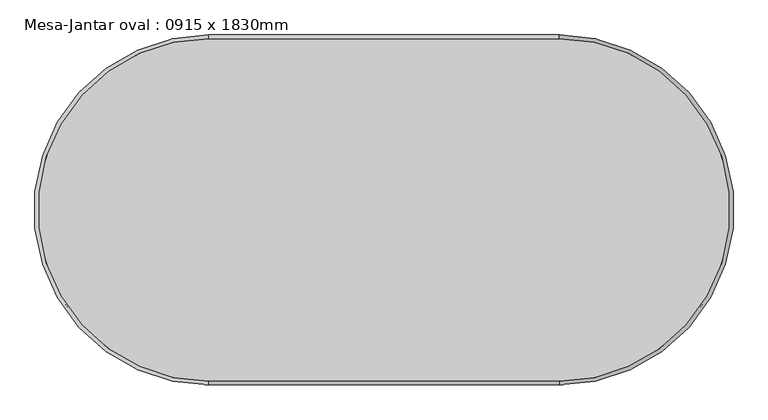
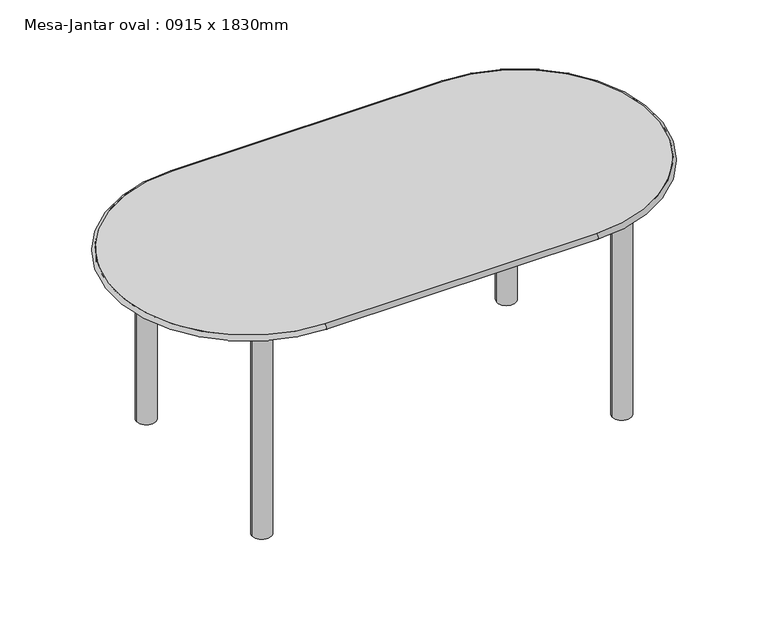
"""IFC4 building model written with IfcOpenShell, lengths in millimetres: furniture geometry, Mesa-Jantar oval : 0915 x 1830mm."""

import ifcopenshell
import ifcopenshell.guid

model = None  # the IFC model being written
_history = None  # IfcOwnerHistory: only IFC2X3 demands one
_inside = {}  # id of a spatial element -> (the spatial element, [elements in it])
_under = {}  # id of a project, library or spatial element -> (it, [spatial elements below it])
_declared = {}  # id of a project -> (the project, [libraries it declares])
_typed = {}  # id of a type object -> (the type object, [elements of that type])
_made_of = {}  # id of a material, layer set ... -> (it, [elements and type objects made of it])


def new_model(schema):
    """Start an empty IFC model of exactly this schema.

    Asked for "IFC4X3", IfcOpenShell would pick the latest addendum, in which some entities
    have other attributes; the version numbers below select the first issue.
    IFC2X3 requires an IfcOwnerHistory on every rooted entity: one is made here for all.
    """
    global model, _history
    if schema == "IFC4X3":
        model = ifcopenshell.file(schema_version=(4, 3, 0, 0))
    else:
        model = ifcopenshell.file(schema=schema)
    _inside.clear()
    _under.clear()
    _declared.clear()
    _typed.clear()
    _made_of.clear()
    _history = None
    if model.schema == "IFC2X3":
        org = make("IfcOrganization", Name="unknown")
        user = make(
            "IfcPersonAndOrganization",
            ThePerson=make("IfcPerson", FamilyName="unknown"),
            TheOrganization=org,
        )
        app = make(
            "IfcApplication",
            ApplicationDeveloper=org,
            Version="unknown",
            ApplicationFullName="unknown",
            ApplicationIdentifier="unknown",
        )
        _history = make(
            "IfcOwnerHistory",
            OwningUser=user,
            OwningApplication=app,
            ChangeAction="ADDED",
            CreationDate=0,
        )
    return model


def make(cls, **values):
    """One entity of the class cls with the attributes given. An attribute that is None is left unset."""
    return model.create_entity(
        cls, **{name: value for name, value in values.items() if value is not None}
    )


def rooted(cls, **values):
    """An entity with a GlobalId (a new one), such as an element, a storey or a relation."""
    return make(cls, GlobalId=ifcopenshell.guid.new(), OwnerHistory=_history, **values)


def si_unit(unit_type, name, prefix=None):
    """IfcSIUnit, for example si_unit("LENGTHUNIT", "METRE", prefix="MILLI")."""
    return make("IfcSIUnit", UnitType=unit_type, Prefix=prefix, Name=name)


def assignment(units):
    """IfcUnitAssignment: the units of a project."""
    return None if units is None else make("IfcUnitAssignment", Units=units)


def point(xyz):
    """IfcCartesianPoint."""
    return None if xyz is None else make("IfcCartesianPoint", Coordinates=xyz)


def direction(xyz):
    """IfcDirection."""
    return None if xyz is None else make("IfcDirection", DirectionRatios=xyz)


def frame(location, z_axis=None, x_axis=None):
    """IfcAxis2Placement3D, a coordinate frame: its origin and axes. An axis left out is left unset."""
    return make(
        "IfcAxis2Placement3D",
        Location=point(location),
        Axis=direction(z_axis),
        RefDirection=direction(x_axis),
    )


def frame_2d(location, x_axis=None):
    """IfcAxis2Placement2D, a coordinate frame in the plane: its origin and x axis."""
    return make(
        "IfcAxis2Placement2D", Location=point(location), RefDirection=direction(x_axis)
    )


def origin():
    """The frame at (0, 0, 0) with its axes left unset."""
    return frame((0.0, 0.0, 0.0))


def origin_with_axes():
    """The frame at (0, 0, 0) with the z axis (0, 0, 1) and the x axis (1, 0, 0) written out."""
    return frame((0.0, 0.0, 0.0), z_axis=(0.0, 0.0, 1.0), x_axis=(1.0, 0.0, 0.0))


def place(relative_to, where):
    """IfcLocalPlacement: puts the frame where relative to a parent placement (None: the world)."""
    return make(
        "IfcLocalPlacement", PlacementRelTo=relative_to, RelativePlacement=where
    )


def context(
    kind, dimensions, precision=None, world=None, true_north=None, identifier=None
):
    """IfcGeometricRepresentationContext, for example the 3D "Model" context."""
    return make(
        "IfcGeometricRepresentationContext",
        ContextIdentifier=identifier,
        ContextType=kind,
        CoordinateSpaceDimension=dimensions,
        Precision=precision,
        WorldCoordinateSystem=world,
        TrueNorth=true_north,
    )


def project(units=None, contexts=None):
    """IfcProject with its units and contexts."""
    return rooted(
        "IfcProject",
        Name="project",
        RepresentationContexts=contexts,
        UnitsInContext=assignment(units),
    )


def spatial(cls, under=None, at=None, **own):
    """A site, building, storey or space (cls), placed at a placement, below another one or the project."""
    s = rooted(cls, ObjectPlacement=at, **own)
    if under is not None:
        _under.setdefault(under.id(), (under, []))[1].append(s)
    return s


def polyline(points):
    """IfcPolyline through the points."""
    return make("IfcPolyline", Points=[point(p) for p in points])


def circle_curve(where, radius):
    """IfcCircle in the frame where."""
    return make("IfcCircle", Position=where, Radius=radius)


def ellipse_curve(where, semi_axis1, semi_axis2):
    """IfcEllipse in the frame where."""
    return make(
        "IfcEllipse", Position=where, SemiAxis1=semi_axis1, SemiAxis2=semi_axis2
    )


def trimmed(basis, trim1, trim2, sense, master):
    """IfcTrimmedCurve: the piece of a basis curve between two trims."""
    return make(
        "IfcTrimmedCurve",
        BasisCurve=basis,
        Trim1=trim1,
        Trim2=trim2,
        SenseAgreement=sense,
        MasterRepresentation=master,
    )


def segment(curve, same_sense, transition):
    """IfcCompositeCurveSegment."""
    return make(
        "IfcCompositeCurveSegment",
        Transition=transition,
        SameSense=same_sense,
        ParentCurve=curve,
    )


def composite_curve(segments, self_intersect=None):
    """IfcCompositeCurve: segments joined end to end."""
    return make("IfcCompositeCurve", Segments=segments, SelfIntersect=self_intersect)


def outline(outer, holes=None, kind="AREA"):
    """IfcArbitraryClosedProfileDef: a profile drawn as a closed curve; with holes, ...WithVoids."""
    if holes is None:
        return make("IfcArbitraryClosedProfileDef", ProfileType=kind, OuterCurve=outer)
    return make(
        "IfcArbitraryProfileDefWithVoids",
        ProfileType=kind,
        OuterCurve=outer,
        InnerCurves=holes,
    )


def extrude(swept, where, along, depth):
    """IfcExtrudedAreaSolid: the profile swept, set in the frame where, extruded along a direction by depth."""
    return make(
        "IfcExtrudedAreaSolid",
        SweptArea=swept,
        Position=where,
        ExtrudedDirection=direction(along),
        Depth=depth,
    )


def shape(context_of_items, identifier, shape_type, items):
    """IfcShapeRepresentation: the items that make up one representation, for example the "Body"."""
    return make(
        "IfcShapeRepresentation",
        ContextOfItems=context_of_items,
        RepresentationIdentifier=identifier,
        RepresentationType=shape_type,
        Items=items,
    )


def source(mapping_origin, context_of_items, identifier, shape_type, items):
    """IfcRepresentationMap: a shape defined once, which mapped items show again and again."""
    return make(
        "IfcRepresentationMap",
        MappingOrigin=mapping_origin,
        MappedRepresentation=shape(context_of_items, identifier, shape_type, items),
    )


def transform(
    local_origin,
    x_axis=None,
    y_axis=None,
    z_axis=None,
    scale=None,
    scale2=None,
    scale3=None,
    uniform=True,
):
    """IfcCartesianTransformationOperator3D, or its non-uniform kind. x_axis, y_axis, z_axis: its Axis1, 2, 3."""
    if uniform:
        return make(
            "IfcCartesianTransformationOperator3D",
            Axis1=direction(x_axis),
            Axis2=direction(y_axis),
            LocalOrigin=point(local_origin),
            Scale=scale,
            Axis3=direction(z_axis),
        )
    return make(
        "IfcCartesianTransformationOperator3DnonUniform",
        Axis1=direction(x_axis),
        Axis2=direction(y_axis),
        LocalOrigin=point(local_origin),
        Scale=scale,
        Axis3=direction(z_axis),
        Scale2=scale2,
        Scale3=scale3,
    )


def mapped(mapping_source, mapping_target):
    """IfcMappedItem: shows the shape of a source again, moved by a transform."""
    return make(
        "IfcMappedItem", MappingSource=mapping_source, MappingTarget=mapping_target
    )


def made_of(thing, what):
    """Note that an element or type object is made of a material, layer set ...; save() writes the relation."""
    if what is not None:
        _made_of.setdefault(what.id(), (what, []))[1].append(thing)
    return thing


def element(
    cls,
    number,
    at=None,
    inside=None,
    cuts=None,
    type_object=None,
    material=None,
    context=None,
    identifier="Body",
    shape_type=None,
    held_by="IfcProductDefinitionShape",
    body=None,
    shapes=None,
    **own,
):
    """One element of the class cls, such as IfcWall. Its Tag is "e" and its number.

    at: its placement. inside: the storey or other place that contains it. cuts: it is an
    opening in that element (IfcRelVoidsElement). A single representation is given by context,
    identifier, shape_type and body (its items); several are given by shapes. held_by: the class
    of the entity that holds the representations. save() writes the other relations.
    """
    e = rooted(cls, Tag="e%d" % number, ObjectPlacement=at, **own)
    if body is not None:
        shapes = [shape(context, identifier, shape_type, body)]
    if shapes is not None:
        e.Representation = make(held_by, Representations=shapes)
    if inside is not None:
        _inside.setdefault(inside.id(), (inside, []))[1].append(e)
    if cuts is not None:
        rooted(
            "IfcRelVoidsElement", RelatingBuildingElement=cuts, RelatedOpeningElement=e
        )
    if type_object is not None:
        _typed.setdefault(type_object.id(), (type_object, []))[1].append(e)
    return made_of(e, material)


def aggregate(whole, parts):
    """IfcRelAggregates: a whole, such as a stair, and the parts it consists of."""
    return rooted("IfcRelAggregates", RelatingObject=whole, RelatedObjects=parts)


def save(model, path):
    """Write the relations noted so far, then the file.

    IfcRelAggregates (storeys below a building ...), IfcRelContainedInSpatialStructure (elements
    in a storey), IfcRelDefinesByType, IfcRelAssociatesMaterial and IfcRelDeclares: one each for
    every whole, place, type object, material and project.
    """
    for whole, parts in _under.values():
        aggregate(whole, parts)
    for where, things in _inside.values():
        rooted(
            "IfcRelContainedInSpatialStructure",
            RelatedElements=things,
            RelatingStructure=where,
        )
    for kind, things in _typed.values():
        rooted("IfcRelDefinesByType", RelatedObjects=things, RelatingType=kind)
    for what, things in _made_of.values():
        rooted("IfcRelAssociatesMaterial", RelatedObjects=things, RelatingMaterial=what)
    for by, libraries in _declared.values():
        rooted("IfcRelDeclares", RelatingContext=by, RelatedDefinitions=libraries)
    model.write(path)


def plane_surface(at):
    """IfcPlane: the flat surface through the origin of the frame at, square to its z axis."""
    return make("IfcPlane", Position=at)


def cylinder_surface(at, radius):
    """IfcCylindricalSurface: all points at the distance radius from the z axis of the frame at."""
    return make("IfcCylindricalSurface", Position=at, Radius=radius)


def revolved_surface(curve, axis_point, axis_direction):
    """IfcSurfaceOfRevolution: the curve turned about the line through axis_point along axis_direction."""
    return make(
        "IfcSurfaceOfRevolution",
        SweptCurve=make("IfcArbitraryOpenProfileDef", ProfileType="CURVE", Curve=curve),
        AxisPosition=make("IfcAxis1Placement", Location=point(axis_point), Axis=direction(axis_direction)),
    )


def advanced_brep(points, edges, surfaces, faces):
    """IfcAdvancedBrep: a solid bounded by faces that lie on surfaces and meet in shared edges.

    An edge is (start, end): straight between two places in points (the first is 0);
    or (start, end, curve); or (start, end, curve, False) where it runs against its curve.
    A face is (place in surfaces, loops), or (place, loops, False) where it looks against
    its surface's normal. A loop lists edges by number (the first is 1), with a minus sign
    where the edge is run from its end to its start. The first loop is the outer one.
    """
    corners = [point(p) for p in points]
    vertices = [make("IfcVertexPoint", VertexGeometry=c) for c in corners]
    made = []
    for start, end, *more in edges:
        made.append(
            make(
                "IfcEdgeCurve",
                EdgeStart=vertices[start],
                EdgeEnd=vertices[end],
                EdgeGeometry=more[0] if more else make("IfcPolyline", Points=[corners[start], corners[end]]),
                SameSense=more[1] if len(more) > 1 else True,
            )
        )
    hull = []
    for where, loops, *sense in faces:
        bounds = []
        for j, loop in enumerate(loops):
            ring = [make("IfcOrientedEdge", EdgeElement=made[abs(k) - 1], Orientation=k > 0) for k in loop]
            bounds.append(
                make(
                    "IfcFaceOuterBound" if j == 0 else "IfcFaceBound",
                    Bound=make("IfcEdgeLoop", EdgeList=ring),
                    Orientation=True,
                )
            )
        hull.append(make("IfcAdvancedFace", Bounds=bounds, FaceSurface=surfaces[where], SameSense=sense[0] if sense else True))
    return make("IfcAdvancedBrep", Outer=make("IfcClosedShell", CfsFaces=hull))


def mesa_jantar_oval_0915_x_1830mm_a7cfbe21(model_context):
    return source(origin(), model_context, "Body", "SolidModel", [
        advanced_brep(
        [(-859.3196721, -806.0733607, 762.0), (-859.3196721, -806.0733607, 742.95), (55.6803279, -806.0733607, 742.95), (55.6803279, -806.0733607, 762.0), (55.6803279, 89.8766393, 762.0), (55.6803279, 89.8766393, 742.95), (-859.3196721, 89.8766393, 742.95), (-859.3196721, 89.8766393, 762.0)],
        [
            (0, 1, circle_curve(frame((-859.3196721, -806.0733607, 752.475), z_axis=(1.0, 0.0, 0.0), x_axis=(0.0, 1.0, 0.0)), 9.525)),
            (1, 2),
            (2, 3, circle_curve(frame((55.6803279, -806.0733607, 752.475), z_axis=(-1.0, 0.0, 0.0), x_axis=(0.0, 1.0, 0.0)), 9.525)),
            (3, 0),
            (1, 0),
            (3, 2),
            (4, 3, circle_curve(frame((55.6803279, -358.0983607, 762.0), z_axis=(0.0, 0.0, -1.0), x_axis=(0.0, -1.0, 0.0)), 447.975)),
            (2, 5, circle_curve(frame((55.6803279, -358.0983607, 742.95), z_axis=(0.0, 0.0, 1.0), x_axis=(0.0, -1.0, 0.0)), 447.975)),
            (5, 4, circle_curve(frame((55.6803279, 89.8766393, 752.475), z_axis=(1.0, 0.0, 0.0), x_axis=(0.0, -1.0, 0.0)), 9.525)),
            (4, 5),
            (5, 6),
            (6, 7, circle_curve(frame((-859.3196721, 89.8766393, 752.475), z_axis=(1.0, 0.0, 0.0), x_axis=(0.0, -1.0, 0.0)), 9.525)),
            (7, 4),
            (7, 6),
            (0, 7, circle_curve(frame((-859.3196721, -358.0983607, 762.0), z_axis=(0.0, 0.0, -1.0), x_axis=(0.0, 1.0, 0.0)), 447.975)),
            (6, 1, circle_curve(frame((-859.3196721, -358.0983607, 742.95), z_axis=(0.0, 0.0, 1.0), x_axis=(0.0, 1.0, 0.0)), 447.975)),
        ],
        [
            cylinder_surface(frame((-859.3196721, -806.0733607, 752.475), z_axis=(-1.0, 0.0, 0.0), x_axis=(0.0, 1.0, 0.0)), 9.525),
            plane_surface(frame((-859.3196721, -806.0733607, 762.0), z_axis=(0.0, 1.0, 0.0), x_axis=(1.0, 0.0, 0.0))),
            revolved_surface(trimmed(ellipse_curve(frame((55.6803279, -806.0733607, 752.475), z_axis=(-1.0, 0.0, 0.0), x_axis=(0.0, 1.0, 0.0)), 9.525, 9.525), [point((55.6803279, -806.0733607, 742.95))], [point((55.6803279, -806.0733607, 762.0))], True, "CARTESIAN"), (55.6803279, -358.0983607, 0.0), (0.0, 0.0, 1.0)),
            revolved_surface(polyline([(55.6803279, -806.0733607, 762.0), (55.6803279, -806.0733607, 742.95)]), (55.6803279, -358.0983607, 0.0), (0.0, 0.0, 1.0)),
            cylinder_surface(frame((55.6803279, 89.8766393, 752.475), z_axis=(1.0, 0.0, 0.0), x_axis=(0.0, -1.0, 0.0)), 9.525),
            plane_surface(frame((55.6803279, 89.8766393, 762.0), z_axis=(0.0, -1.0, 0.0), x_axis=(-1.0, 0.0, 0.0))),
            revolved_surface(trimmed(ellipse_curve(frame((-859.3196721, 89.8766393, 752.475), z_axis=(1.0, 0.0, 0.0), x_axis=(0.0, -1.0, 0.0)), 9.525, 9.525), [point((-859.3196721, 89.8766393, 742.95))], [point((-859.3196721, 89.8766393, 762.0))], True, "CARTESIAN"), (-859.3196721, -358.0983607, 0.0), (0.0, 0.0, 1.0)),
            revolved_surface(polyline([(-859.3196721, 89.87663930000002, 762.0), (-859.3196721, 89.87663930000002, 742.95)]), (-859.3196721, -358.0983607, 0.0), (0.0, 0.0, 1.0)),
        ],
        [
            (0, [[1, 2, 3, 4]]),
            (1, [[5, -4, 6, -2]]),
            (2, [[7, -3, 8, 9]]),
            (3, [[-8, -6, -7, 10]]),
            (4, [[-9, 11, 12, 13]]),
            (5, [[-10, -13, 14, -11]]),
            (6, [[15, -12, 16, -1]]),
            (7, [[-16, -14, -15, -5]]),
        ],
    ),
        extrude(outline(composite_curve([segment(trimmed(circle_curve(frame_2d((-1008.5446721, -21.2483607)), 31.75), [point((-1040.2946721, -21.2483607))], [point((-976.7946721, -21.2483607))], False, "CARTESIAN"), True, "CONTINUOUS"), segment(trimmed(circle_curve(frame_2d((-1008.5446721, -21.2483607)), 31.75), [point((-976.7946721, -21.2483607))], [point((-1040.2946721, -21.2483607))], False, "CARTESIAN"), True, "CONTINUOUS")], self_intersect=False)), origin_with_axes(), (0.0, 0.0, 1.0), 742.95),
        extrude(outline(composite_curve([segment(trimmed(circle_curve(frame_2d((-1008.5446721, -694.9483607)), 31.75), [point((-1040.2946721, -694.9483607))], [point((-976.7946721, -694.9483607))], False, "CARTESIAN"), True, "CONTINUOUS"), segment(trimmed(circle_curve(frame_2d((-1008.5446721, -694.9483607)), 31.75), [point((-976.7946721, -694.9483607))], [point((-1040.2946721, -694.9483607))], False, "CARTESIAN"), True, "CONTINUOUS")], self_intersect=False)), origin_with_axes(), (0.0, 0.0, 1.0), 742.95),
        extrude(outline(composite_curve([segment(trimmed(circle_curve(frame_2d((204.9053279, -21.2483607)), 31.75), [point((173.1553279, -21.2483607))], [point((236.6553279, -21.2483607))], False, "CARTESIAN"), True, "CONTINUOUS"), segment(trimmed(circle_curve(frame_2d((204.9053279, -21.2483607)), 31.75), [point((236.6553279, -21.2483607))], [point((173.1553279, -21.2483607))], False, "CARTESIAN"), True, "CONTINUOUS")], self_intersect=False)), origin_with_axes(), (0.0, 0.0, 1.0), 742.95),
        extrude(outline(composite_curve([segment(trimmed(circle_curve(frame_2d((204.9053279, -694.9483607)), 31.75), [point((173.1553279, -694.9483607))], [point((236.6553279, -694.9483607))], False, "CARTESIAN"), True, "CONTINUOUS"), segment(trimmed(circle_curve(frame_2d((204.9053279, -694.9483607)), 31.75), [point((236.6553279, -694.9483607))], [point((173.1553279, -694.9483607))], False, "CARTESIAN"), True, "CONTINUOUS")], self_intersect=False)), origin_with_axes(), (0.0, 0.0, 1.0), 742.95),
        extrude(outline(polyline([(223.9553279, -2.1983607), (223.9553279, -713.9983607), (-1027.5946721, -713.9983607), (-1027.5946721, -2.1983607), (223.9553279, -2.1983607)]), holes=[polyline([(204.9053279, -21.2483607), (-1008.5446721, -21.2483607), (-1008.5446721, -694.9483607), (204.9053279, -694.9483607), (204.9053279, -21.2483607)])]), frame((0.0, 0.0, 692.15), z_axis=(0.0, 0.0, 1.0), x_axis=(1.0, 0.0, 0.0)), (0.0, 0.0, 1.0), 50.8),
        extrude(outline(composite_curve([segment(polyline([(-859.3196721, 89.8766393), (55.6803279, 89.8766393)]), True, "CONTINUOUS"), segment(trimmed(circle_curve(frame_2d((55.6803279, -358.0983607)), 447.975), [point((55.6803279, 89.8766393))], [point((503.6553279, -358.0983607))], False, "CARTESIAN"), True, "CONTINUOUS"), segment(trimmed(circle_curve(frame_2d((55.6803279, -358.0983607)), 447.975), [point((503.6553279, -358.0983607))], [point((55.6803279, -806.0733607))], False, "CARTESIAN"), True, "CONTINUOUS"), segment(polyline([(55.6803279, -806.0733607), (-859.3196721, -806.0733607)]), True, "CONTINUOUS"), segment(trimmed(circle_curve(frame_2d((-859.3196721, -358.0983607)), 447.975), [point((-859.3196721, -806.0733607))], [point((-1307.2946721, -358.0983607))], False, "CARTESIAN"), True, "CONTINUOUS"), segment(trimmed(circle_curve(frame_2d((-859.3196721, -358.0983607)), 447.975), [point((-1307.2946721, -358.0983607))], [point((-859.3196721, 89.8766393))], False, "CARTESIAN"), True, "CONTINUOUS")], self_intersect=False)), frame((0.0, 0.0, 742.95), z_axis=(0.0, 0.0, 1.0), x_axis=(1.0, 0.0, 0.0)), (0.0, 0.0, 1.0), 19.05),
    ])


if __name__ == "__main__":
    model = new_model("IFC4")
    model_context = context("Model", 3, world=origin())
    ifc_project = project(units=[si_unit("LENGTHUNIT", "METRE", prefix="MILLI")], contexts=[model_context])
    site = spatial("IfcSite", under=ifc_project)
    building = spatial("IfcBuilding", under=site)
    placement = place(None, origin())
    mesa_jantar_oval_0915_x_1830mm_shape = mesa_jantar_oval_0915_x_1830mm_a7cfbe21(model_context)
    element("IfcFurniture", 1, ObjectType="Mesa-Jantar oval : 0915 x 1830mm", at=placement, inside=building, context=model_context, shape_type="MappedRepresentation", body=[
        mapped(mesa_jantar_oval_0915_x_1830mm_shape, transform((0.0, 0.0, 0.0), x_axis=(1.0, 0.0, 0.0), y_axis=(0.0, 1.0, 0.0), z_axis=(0.0, 0.0, 1.0))),
    ])
    save(model, "model.ifc")

# Revit data of these elements
# Type "Mesa-Jantar oval : 0915 x 1830mm"
#   Comprimento = 1830 mm
#   Largura = 915 mm
#   Material base = none
#   Material superior = none
# Element 1 (IfcFurniture, "Mesa-Jantar oval : 0915 x 1830mm")
#   Materials on its faces: "Vidro - Claro, Cinza"
# Materials
#   "Vidro - Claro, Cinza": class "Vidro", colour RGB 252 255 255, transparency 0.64
